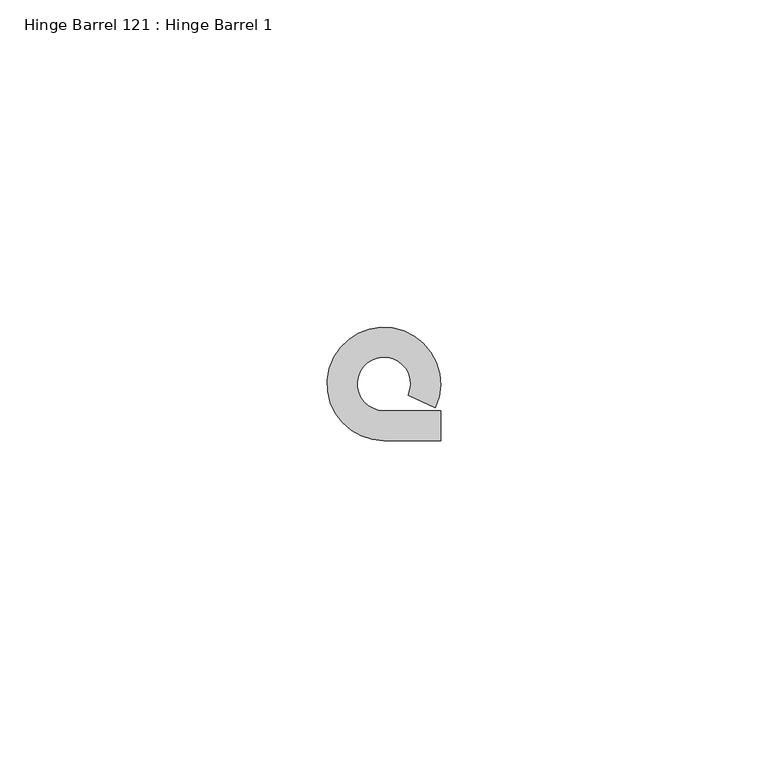
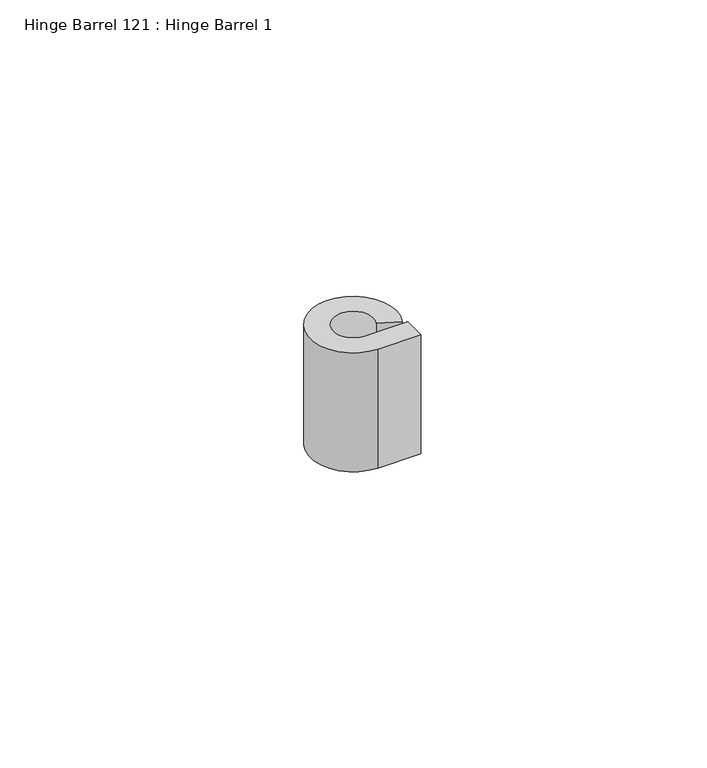
"""IFC4 building model written with IfcOpenShell, lengths in millimetres: proxy geometry, Hinge Barrel 121 : Hinge Barrel 1."""

from ifc_helpers import new_model, si_unit, point, frame, frame_2d, origin, place, context, project, spatial, polyline, circle_curve, trimmed, segment, composite_curve, outline, extrude, source, transform, mapped, element, save


def hinge_barrel_121_hinge_barrel_1_b6c159eb(model_context):
    return source(origin(), model_context, "Body", "SweptSolid", [
        extrude(outline(composite_curve([segment(polyline([(587323.2214739, -534104.7943841), (587327.7934739, -534104.7943841), (587327.7934739, -534109.3584466), (587319.1320739, -534109.3584466)]), True, "CONTINUOUS"), segment(trimmed(circle_curve(frame_2d((587319.1320739, -534100.7049841)), 8.6534625), [point((587319.1320739, -534109.3584466))], [point((587326.986084, -534104.3377433))], False, "CARTESIAN"), True, "CONTINUOUS"), segment(polyline([(587326.986084, -534104.3377433), (587322.8436736, -534102.421731)]), True, "CONTINUOUS"), segment(trimmed(circle_curve(frame_2d((587319.1320739, -534100.7049841)), 4.0894), [point((587322.8436736, -534102.421731))], [point((587319.1320739, -534104.7943841))], True, "CARTESIAN"), True, "CONTINUOUS"), segment(polyline([(587319.1320739, -534104.7943841), (587323.2214739, -534104.7943841)]), True, "CONTINUOUS")], self_intersect=False)), frame((0.0, 0.0, 1123.95), z_axis=(0.0, 0.0, 1.0), x_axis=(1.0, 0.0, 0.0)), (0.0, 0.0, 1.0), 25.4),
    ])


if __name__ == "__main__":
    model = new_model("IFC4")
    model_context = context("Model", 3, world=origin())
    ifc_project = project(units=[si_unit("LENGTHUNIT", "METRE", prefix="MILLI")], contexts=[model_context])
    site = spatial("IfcSite", under=ifc_project)
    building = spatial("IfcBuilding", under=site)
    placement = place(None, origin())
    hinge_barrel_121_hinge_barrel_1_shape = hinge_barrel_121_hinge_barrel_1_b6c159eb(model_context)
    element("IfcBuildingElementProxy", 1, Name="Hinge Barrel 121 : Hinge Barrel 1", ObjectType="Hinge Barrel 121 : Hinge Barrel 1", at=placement, inside=building, context=model_context, shape_type="MappedRepresentation", body=[
        mapped(hinge_barrel_121_hinge_barrel_1_shape, transform((0.0, 0.0, 0.0), x_axis=(1.0, 0.0, 0.0), y_axis=(0.0, 1.0, 0.0), z_axis=(0.0, 0.0, 1.0))),
    ])
    save(model, "model.ifc")

# Revit data of these elements
# Element 1 (IfcBuildingElementProxy, "Hinge Barrel 121 : Hinge Barrel 1")
#   Materials on its faces: "6\"X6\" WELD-ON STL BUTT HINGE"
# Materials
#   "6\"X6\" WELD-ON STL BUTT HINGE": class "Metal", colour RGB 189 187 185, transparency 0, Description = "Carbon steel", Cost = 0
